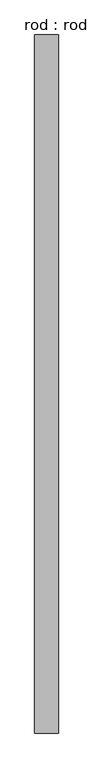
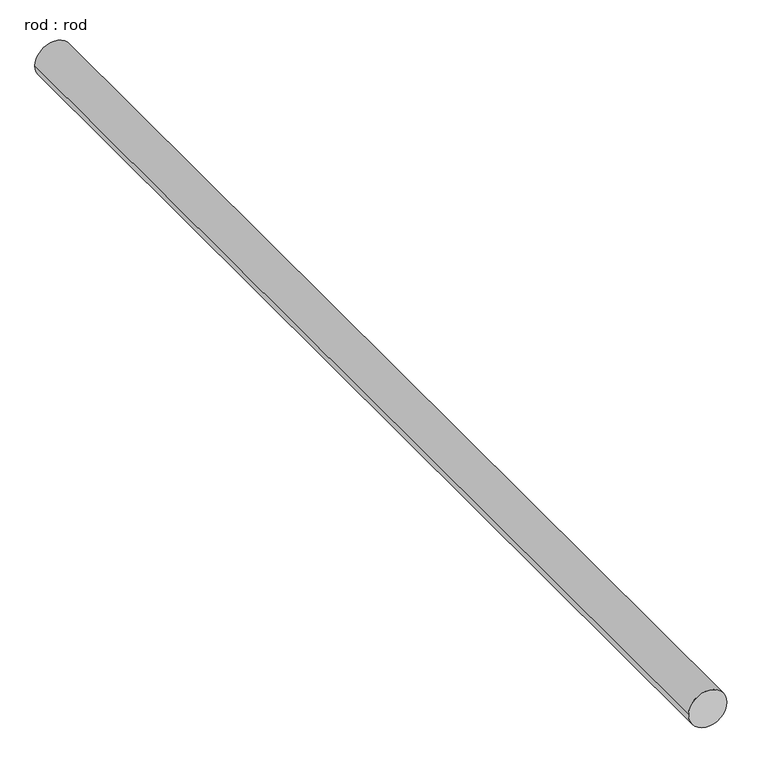
"""IFC4 building model written with IfcOpenShell, lengths in millimetres: proxy geometry, rod : rod."""

from ifc_helpers import new_model, si_unit, point, frame, frame_2d, origin, place, context, project, spatial, circle_curve, trimmed, segment, composite_curve, outline, extrude, source, transform, mapped, element, save


def rod_rod_68d13460(model_context):
    return source(origin(), model_context, "Body", "SweptSolid", [
        extrude(outline(composite_curve([segment(trimmed(circle_curve(frame_2d((0.0108462, 0.0)), 200.0), [point((0.0108462, 200.0))], [point((0.0108462, -200.0))], False, "CARTESIAN"), True, "CONTINUOUS"), segment(trimmed(circle_curve(frame_2d((0.0108462, 0.0)), 200.0), [point((0.0108462, -200.0))], [point((0.0108462, 200.0))], False, "CARTESIAN"), True, "CONTINUOUS")], self_intersect=False)), frame((0.0, -1825.2000958, 0.0), z_axis=(0.0, 1.0, 0.0), x_axis=(0.0, 0.0, 1.0)), (0.0, 0.0, 1.0), 11835.8574222),
    ])


if __name__ == "__main__":
    model = new_model("IFC4")
    model_context = context("Model", 3, world=origin())
    ifc_project = project(units=[si_unit("LENGTHUNIT", "METRE", prefix="MILLI")], contexts=[model_context])
    site = spatial("IfcSite", under=ifc_project)
    building = spatial("IfcBuilding", under=site)
    placement = place(None, origin())
    rod_rod_shape = rod_rod_68d13460(model_context)
    element("IfcBuildingElementProxy", 1, Name="rod : rod", ObjectType="rod : rod", at=placement, inside=building, context=model_context, shape_type="MappedRepresentation", body=[
        mapped(rod_rod_shape, transform((0.0, 0.0, 0.0), x_axis=(1.0, 0.0, 0.0), y_axis=(0.0, 1.0, 0.0), z_axis=(0.0, 0.0, 1.0))),
    ])
    save(model, "model.ifc")

# Revit data of these elements
# Type "rod : rod"
#   Default Elevation = 0
